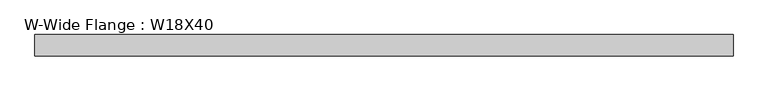
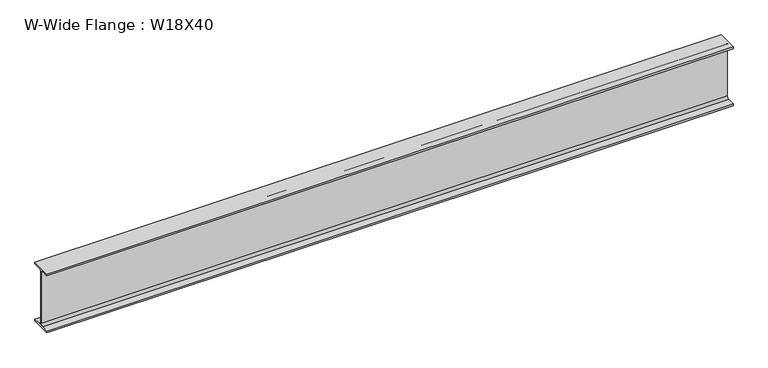
"""IFC4 building model written with IfcOpenShell, lengths in millimetres: beam geometry, W-Wide Flange : W18X40."""

from ifc_helpers import new_model, si_unit, point, frame, frame_2d, origin, place, context, project, spatial, polyline, circle_curve, trimmed, segment, composite_curve, outline, extrude, source, transform, mapped, element, save


def w_wide_flange_w18x40_88806548(model_context):
    return source(origin(), model_context, "Body", "SweptSolid", [
        extrude(outline(composite_curve([segment(polyline([(76.454, -213.995), (76.454, -227.33), (-76.454, -227.33), (-76.454, -213.995), (-20.828, -213.995)]), True, "CONTINUOUS"), segment(trimmed(circle_curve(frame_2d((-20.828, -197.1675)), 16.8275), [point((-20.828, -213.995))], [point((-4.0005, -197.1675))], True, "CARTESIAN"), True, "CONTINUOUS"), segment(polyline([(-4.0005, -197.1675), (-4.0005, 197.1675)]), True, "CONTINUOUS"), segment(trimmed(circle_curve(frame_2d((-20.828, 197.1675)), 16.8275), [point((-4.0005, 197.1675))], [point((-20.828, 213.995))], True, "CARTESIAN"), True, "CONTINUOUS"), segment(polyline([(-20.828, 213.995), (-76.454, 213.995), (-76.454, 227.33), (76.454, 227.33), (76.454, 213.995), (20.828, 213.995)]), True, "CONTINUOUS"), segment(trimmed(circle_curve(frame_2d((20.828, 197.1675)), 16.8275), [point((20.828, 213.995))], [point((4.0005, 197.1675))], True, "CARTESIAN"), True, "CONTINUOUS"), segment(polyline([(4.0005, 197.1675), (4.0005, -197.1675)]), True, "CONTINUOUS"), segment(trimmed(circle_curve(frame_2d((20.828, -197.1675)), 16.8275), [point((4.0005, -197.1675))], [point((20.828, -213.995))], True, "CARTESIAN"), True, "CONTINUOUS"), segment(polyline([(20.828, -213.995), (76.454, -213.995)]), True, "CONTINUOUS")], self_intersect=False)), frame((-2514.6, 0.0, 0.0), z_axis=(1.0, 0.0, 0.0), x_axis=(0.0, 1.0, 0.0)), (0.0, 0.0, 1.0), 5029.2),
    ])


if __name__ == "__main__":
    model = new_model("IFC4")
    model_context = context("Model", 3, world=origin())
    ifc_project = project(units=[si_unit("LENGTHUNIT", "METRE", prefix="MILLI")], contexts=[model_context])
    site = spatial("IfcSite", under=ifc_project)
    building = spatial("IfcBuilding", under=site)
    placement = place(None, origin())
    w_wide_flange_w18x40_shape = w_wide_flange_w18x40_88806548(model_context)
    element("IfcBeam", 1, ObjectType="W-Wide Flange : W18X40", at=placement, inside=building, context=model_context, shape_type="MappedRepresentation", body=[
        mapped(w_wide_flange_w18x40_shape, transform((0.0, 0.0, 0.0), x_axis=(1.0, 0.0, 0.0), y_axis=(0.0, 1.0, 0.0), z_axis=(0.0, 0.0, 1.0))),
    ])
    save(model, "model.ifc")

# Revit data of these elements
# Type "W-Wide Flange : W18X40"
#   Assembly Code = "B10"
#   W = 40
#   Length [instance default] = 5' - 0"
#   bf = 0' - 6.02"
#   d = 1' - 5.9"
#   k = 0' - 1 3/16"
#   k2 = 0' - 0.6625"
#   tf = 0' - 0.525"
#   tw = 0' - 0.315"
#   A = 0.0819444 SF
#   Structural Material [instance default] = Steel ASTM A992
# Element 1 (IfcBeam, "W-Wide Flange : W18X40")
#   Materials on its faces: "Steel ASTM A992"
# Materials
#   "Steel ASTM A992": class "Metal", colour RGB 199 199 199, transparency 0, Description = "Structural steel 50ksi", Cost = 0
